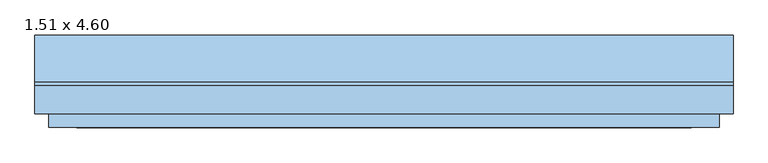
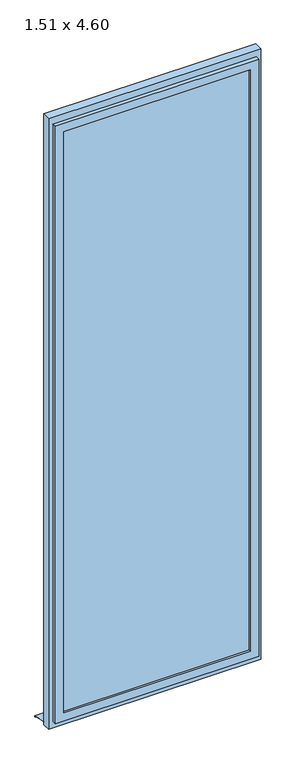
"""IFC4 building model written with IfcOpenShell, lengths in millimetres: window geometry, Fenstertür 1-flg : 1.51 x 4.60."""

import ifcopenshell
import ifcopenshell.guid

model = None  # the IFC model being written
_history = None  # IfcOwnerHistory: only IFC2X3 demands one
_inside = {}  # id of a spatial element -> (the spatial element, [elements in it])
_under = {}  # id of a project, library or spatial element -> (it, [spatial elements below it])
_declared = {}  # id of a project -> (the project, [libraries it declares])
_typed = {}  # id of a type object -> (the type object, [elements of that type])
_made_of = {}  # id of a material, layer set ... -> (it, [elements and type objects made of it])


def new_model(schema):
    """Start an empty IFC model of exactly this schema.

    Asked for "IFC4X3", IfcOpenShell would pick the latest addendum, in which some entities
    have other attributes; the version numbers below select the first issue.
    IFC2X3 requires an IfcOwnerHistory on every rooted entity: one is made here for all.
    """
    global model, _history
    if schema == "IFC4X3":
        model = ifcopenshell.file(schema_version=(4, 3, 0, 0))
    else:
        model = ifcopenshell.file(schema=schema)
    _inside.clear()
    _under.clear()
    _declared.clear()
    _typed.clear()
    _made_of.clear()
    _history = None
    if model.schema == "IFC2X3":
        org = make("IfcOrganization", Name="unknown")
        user = make(
            "IfcPersonAndOrganization",
            ThePerson=make("IfcPerson", FamilyName="unknown"),
            TheOrganization=org,
        )
        app = make(
            "IfcApplication",
            ApplicationDeveloper=org,
            Version="unknown",
            ApplicationFullName="unknown",
            ApplicationIdentifier="unknown",
        )
        _history = make(
            "IfcOwnerHistory",
            OwningUser=user,
            OwningApplication=app,
            ChangeAction="ADDED",
            CreationDate=0,
        )
    return model


def make(cls, **values):
    """One entity of the class cls with the attributes given. An attribute that is None is left unset."""
    return model.create_entity(
        cls, **{name: value for name, value in values.items() if value is not None}
    )


def rooted(cls, **values):
    """An entity with a GlobalId (a new one), such as an element, a storey or a relation."""
    return make(cls, GlobalId=ifcopenshell.guid.new(), OwnerHistory=_history, **values)


def si_unit(unit_type, name, prefix=None):
    """IfcSIUnit, for example si_unit("LENGTHUNIT", "METRE", prefix="MILLI")."""
    return make("IfcSIUnit", UnitType=unit_type, Prefix=prefix, Name=name)


def assignment(units):
    """IfcUnitAssignment: the units of a project."""
    return None if units is None else make("IfcUnitAssignment", Units=units)


def point(xyz):
    """IfcCartesianPoint."""
    return None if xyz is None else make("IfcCartesianPoint", Coordinates=xyz)


def direction(xyz):
    """IfcDirection."""
    return None if xyz is None else make("IfcDirection", DirectionRatios=xyz)


def frame(location, z_axis=None, x_axis=None):
    """IfcAxis2Placement3D, a coordinate frame: its origin and axes. An axis left out is left unset."""
    return make(
        "IfcAxis2Placement3D",
        Location=point(location),
        Axis=direction(z_axis),
        RefDirection=direction(x_axis),
    )


def origin():
    """The frame at (0, 0, 0) with its axes left unset."""
    return frame((0.0, 0.0, 0.0))


def place(relative_to, where):
    """IfcLocalPlacement: puts the frame where relative to a parent placement (None: the world)."""
    return make(
        "IfcLocalPlacement", PlacementRelTo=relative_to, RelativePlacement=where
    )


def context(
    kind, dimensions, precision=None, world=None, true_north=None, identifier=None
):
    """IfcGeometricRepresentationContext, for example the 3D "Model" context."""
    return make(
        "IfcGeometricRepresentationContext",
        ContextIdentifier=identifier,
        ContextType=kind,
        CoordinateSpaceDimension=dimensions,
        Precision=precision,
        WorldCoordinateSystem=world,
        TrueNorth=true_north,
    )


def project(units=None, contexts=None):
    """IfcProject with its units and contexts."""
    return rooted(
        "IfcProject",
        Name="project",
        RepresentationContexts=contexts,
        UnitsInContext=assignment(units),
    )


def spatial(cls, under=None, at=None, **own):
    """A site, building, storey or space (cls), placed at a placement, below another one or the project."""
    s = rooted(cls, ObjectPlacement=at, **own)
    if under is not None:
        _under.setdefault(under.id(), (under, []))[1].append(s)
    return s


def polyline(points):
    """IfcPolyline through the points."""
    return make("IfcPolyline", Points=[point(p) for p in points])


def outline(outer, holes=None, kind="AREA"):
    """IfcArbitraryClosedProfileDef: a profile drawn as a closed curve; with holes, ...WithVoids."""
    if holes is None:
        return make("IfcArbitraryClosedProfileDef", ProfileType=kind, OuterCurve=outer)
    return make(
        "IfcArbitraryProfileDefWithVoids",
        ProfileType=kind,
        OuterCurve=outer,
        InnerCurves=holes,
    )


def extrude(swept, where, along, depth):
    """IfcExtrudedAreaSolid: the profile swept, set in the frame where, extruded along a direction by depth."""
    return make(
        "IfcExtrudedAreaSolid",
        SweptArea=swept,
        Position=where,
        ExtrudedDirection=direction(along),
        Depth=depth,
    )


def faces_of(points, faces, orient=None, outer=None):
    """IfcFace entities. A face is a list of loops; a loop is a list of indices into points, from 0.

    orient and outer hold one flag for each loop. By default every Orientation is true, the
    first loop of a face is its IfcFaceOuterBound and the others are IfcFaceBound.
    """
    made = []
    for i, loops in enumerate(faces):
        bounds = []
        for j, loop in enumerate(loops):
            is_outer = j == 0 if outer is None else outer[i][j]
            bounds.append(
                make(
                    "IfcFaceOuterBound" if is_outer else "IfcFaceBound",
                    Bound=make("IfcPolyLoop", Polygon=[points[k] for k in loop]),
                    Orientation=True if orient is None else orient[i][j],
                )
            )
        made.append(make("IfcFace", Bounds=bounds))
    return made


def faceted_brep(points, faces, orient=None, outer=None, voids=None):
    """IfcFacetedBrep: a solid bounded by flat faces; with voids (closed shells), ...WithVoids."""
    shared = [point(p) for p in points]
    hull = make("IfcClosedShell", CfsFaces=faces_of(shared, faces, orient, outer))
    if voids is None:
        return make("IfcFacetedBrep", Outer=hull)
    return make(
        "IfcFacetedBrepWithVoids",
        Outer=hull,
        Voids=[
            make(cls, CfsFaces=faces_of(shared, fs, o, b)) for cls, fs, o, b in voids
        ],
    )


def shape(context_of_items, identifier, shape_type, items):
    """IfcShapeRepresentation: the items that make up one representation, for example the "Body"."""
    return make(
        "IfcShapeRepresentation",
        ContextOfItems=context_of_items,
        RepresentationIdentifier=identifier,
        RepresentationType=shape_type,
        Items=items,
    )


def source(mapping_origin, context_of_items, identifier, shape_type, items):
    """IfcRepresentationMap: a shape defined once, which mapped items show again and again."""
    return make(
        "IfcRepresentationMap",
        MappingOrigin=mapping_origin,
        MappedRepresentation=shape(context_of_items, identifier, shape_type, items),
    )


def transform(
    local_origin,
    x_axis=None,
    y_axis=None,
    z_axis=None,
    scale=None,
    scale2=None,
    scale3=None,
    uniform=True,
):
    """IfcCartesianTransformationOperator3D, or its non-uniform kind. x_axis, y_axis, z_axis: its Axis1, 2, 3."""
    if uniform:
        return make(
            "IfcCartesianTransformationOperator3D",
            Axis1=direction(x_axis),
            Axis2=direction(y_axis),
            LocalOrigin=point(local_origin),
            Scale=scale,
            Axis3=direction(z_axis),
        )
    return make(
        "IfcCartesianTransformationOperator3DnonUniform",
        Axis1=direction(x_axis),
        Axis2=direction(y_axis),
        LocalOrigin=point(local_origin),
        Scale=scale,
        Axis3=direction(z_axis),
        Scale2=scale2,
        Scale3=scale3,
    )


def mapped(mapping_source, mapping_target):
    """IfcMappedItem: shows the shape of a source again, moved by a transform."""
    return make(
        "IfcMappedItem", MappingSource=mapping_source, MappingTarget=mapping_target
    )


def made_of(thing, what):
    """Note that an element or type object is made of a material, layer set ...; save() writes the relation."""
    if what is not None:
        _made_of.setdefault(what.id(), (what, []))[1].append(thing)
    return thing


def element(
    cls,
    number,
    at=None,
    inside=None,
    cuts=None,
    type_object=None,
    material=None,
    context=None,
    identifier="Body",
    shape_type=None,
    held_by="IfcProductDefinitionShape",
    body=None,
    shapes=None,
    **own,
):
    """One element of the class cls, such as IfcWall. Its Tag is "e" and its number.

    at: its placement. inside: the storey or other place that contains it. cuts: it is an
    opening in that element (IfcRelVoidsElement). A single representation is given by context,
    identifier, shape_type and body (its items); several are given by shapes. held_by: the class
    of the entity that holds the representations. save() writes the other relations.
    """
    e = rooted(cls, Tag="e%d" % number, ObjectPlacement=at, **own)
    if body is not None:
        shapes = [shape(context, identifier, shape_type, body)]
    if shapes is not None:
        e.Representation = make(held_by, Representations=shapes)
    if inside is not None:
        _inside.setdefault(inside.id(), (inside, []))[1].append(e)
    if cuts is not None:
        rooted(
            "IfcRelVoidsElement", RelatingBuildingElement=cuts, RelatedOpeningElement=e
        )
    if type_object is not None:
        _typed.setdefault(type_object.id(), (type_object, []))[1].append(e)
    return made_of(e, material)


def aggregate(whole, parts):
    """IfcRelAggregates: a whole, such as a stair, and the parts it consists of."""
    return rooted("IfcRelAggregates", RelatingObject=whole, RelatedObjects=parts)


def save(model, path):
    """Write the relations noted so far, then the file.

    IfcRelAggregates (storeys below a building ...), IfcRelContainedInSpatialStructure (elements
    in a storey), IfcRelDefinesByType, IfcRelAssociatesMaterial and IfcRelDeclares: one each for
    every whole, place, type object, material and project.
    """
    for whole, parts in _under.values():
        aggregate(whole, parts)
    for where, things in _inside.values():
        rooted(
            "IfcRelContainedInSpatialStructure",
            RelatedElements=things,
            RelatingStructure=where,
        )
    for kind, things in _typed.values():
        rooted("IfcRelDefinesByType", RelatedObjects=things, RelatingType=kind)
    for what, things in _made_of.values():
        rooted("IfcRelAssociatesMaterial", RelatedObjects=things, RelatingMaterial=what)
    for by, libraries in _declared.values():
        rooted("IfcRelDeclares", RelatingContext=by, RelatedDefinitions=libraries)
    model.write(path)


def window_1_51_x_4_60_b399f2d8(model_context):
    return source(origin(), model_context, "Body", "SolidModel", [
        extrude(outline(polyline([(4600.0, 755.0), (4600.0, -755.0), (0.0, -755.0), (0.0, 755.0), (4600.0, 755.0)]), holes=[polyline([(4520.0, 695.0), (80.0, 695.0), (80.0, -695.0), (4520.0, -695.0), (4520.0, 695.0)])]), frame((0.0, -80.0, 0.0), z_axis=(0.0, 1.0, 0.0), x_axis=(0.0, 0.0, 1.0)), (0.0, 0.0, 1.0), 60.0),
        faceted_brep([(725.0, -80.0, 4550.0), (725.0, -110.0, 4550.0), (725.0, -110.0, 50.0), (725.0, -80.0, 50.0), (-725.0, -110.0, 4550.0), (-725.0, -110.0, 50.0), (665.0, -110.0, 110.0), (-665.0, -110.0, 110.0), (-665.0, -110.0, 4490.0), (665.0, -110.0, 4490.0), (-725.0, -80.0, 50.0), (-725.0, -80.0, 4550.0), (695.0, -80.0, 4520.0), (-695.0, -80.0, 4520.0), (-695.0, -80.0, 80.0), (695.0, -80.0, 80.0), (695.0, -50.0, 4520.0), (695.0, -50.0, 80.0), (-695.0, -50.0, 80.0), (-695.0, -50.0, 4520.0), (665.0, -50.0, 4490.0), (-665.0, -50.0, 4490.0), (-665.0, -50.0, 110.0), (665.0, -50.0, 110.0)], [[[0, 1, 2, 3]], [[1, 4, 5, 2], [6, 7, 8, 9]], [[3, 2, 5, 10]], [[3, 10, 11, 0], [12, 13, 14, 15]], [[16, 12, 15, 17]], [[17, 15, 14, 18]], [[17, 18, 19, 16], [20, 21, 22, 23]], [[9, 20, 23, 6]], [[6, 23, 22, 7]], [[10, 5, 4, 11]], [[18, 14, 13, 19]], [[7, 22, 21, 8]], [[11, 4, 1, 0]], [[19, 13, 12, 16]], [[8, 21, 20, 9]]]),
        extrude(outline(polyline([(-9.9778457, 20.0), (90.0, 0.0), (90.0, -10.0), (88.0, -10.0), (88.0, -1.6395366), (-10.1759277, 18.0), (-20.0, 18.0), (-20.0, 20.0), (-9.9778457, 20.0)])), frame((-755.0, 0.0, 0.0), z_axis=(1.0, 0.0, 0.0), x_axis=(0.0, 1.0, 0.0)), (0.0, 0.0, 1.0), 1510.0),
        extrude(outline(polyline([(665.0, -95.0), (-665.0, -95.0), (-665.0, -65.0), (665.0, -65.0), (665.0, -95.0)])), frame((0.0, 0.0, 110.0), z_axis=(0.0, 0.0, 1.0), x_axis=(1.0, 0.0, 0.0)), (0.0, 0.0, 1.0), 4380.0),
    ])


if __name__ == "__main__":
    model = new_model("IFC4")
    model_context = context("Model", 3, world=origin())
    ifc_project = project(units=[si_unit("LENGTHUNIT", "METRE", prefix="MILLI")], contexts=[model_context])
    site = spatial("IfcSite", under=ifc_project)
    building = spatial("IfcBuilding", under=site)
    placement = place(None, origin())
    window_1_51_x_4_60_shape = window_1_51_x_4_60_b399f2d8(model_context)
    element("IfcWindow", 1, ObjectType="Fenstertür 1-flg : 1.51 x 4.60", at=placement, inside=building, context=model_context, shape_type="MappedRepresentation", body=[
        mapped(window_1_51_x_4_60_shape, transform((0.0, 0.0, 0.0), x_axis=(1.0, 0.0, 0.0), y_axis=(0.0, 1.0, 0.0), z_axis=(0.0, 0.0, 1.0))),
    ])
    save(model, "model.ifc")

# Revit data of these elements
# Type "Fenstertür 1-flg : 1.51 x 4.60"
#   Type Mark = "59"
#   Operation = "SinglePanel"
#   Construction Type Id = "SGL"
#   Keynote = "16.05.01"
#   Analytic Construction = "Große Fenster mit Einfachverglasung"
#   Visual Light Transmittance = 0.9
#   Solar Heat Gain Coefficient = 0.86
#   Rough Width = 1.510 m
#   Rough Height = 4.600 m
#   Heat Transfer Coefficient (U) = 5.5617 W/(m²·K)
#   Rahmentiefe = 0.060 m
#   Rahmenhöhe unten = 0.080 m
#   Höhe oberer  Rahmen = 0.080 m
#   Rahmenbreite = 0.060 m
#   Height = 4.600 m
#   Tiefe Flügel = 0.060 m
#   Flügelbreite = 0.060 m
#   Einbautiefe (von außen) [instance default] = 0.080 m
#   Width = 1.510 m
#   Sichtbarkeit Sturzlinien [instance default] = yes
#   Öffnungsrichtung oben [instance default] = yes
#   Öffnungsrichtung in Draufsicht anzeigen [instance default] = yes
#   Drehflügel 1 [instance default] = yes
#   Bild [instance default] = none
#   Glas [instance default] = none
#   Fensterflügel [instance default] = none
#   Äußere Fensterbank [instance default] = none
#   Wall Closure = (empty or 0)
# Element 1 (IfcWindow, "Fenstertür 1-flg : 1.51 x 4.60")
#   Materials on its faces: "Kunststoff - Weiß", "Glas"
# Materials
#   "Kunststoff - Weiß": class "Kunststoff", colour RGB 249 249 249, transparency 0, Cost = 0
#   "Glas": class "Glas", colour RGB 0 0 255, transparency 0.75, Comments = "Render-Darstellung nicht aktualisiert ", Cost = 0
